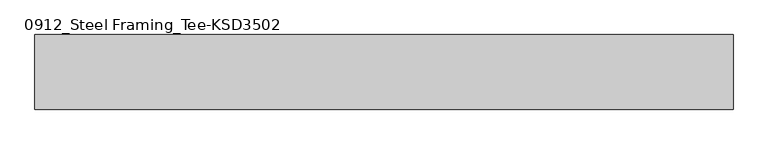
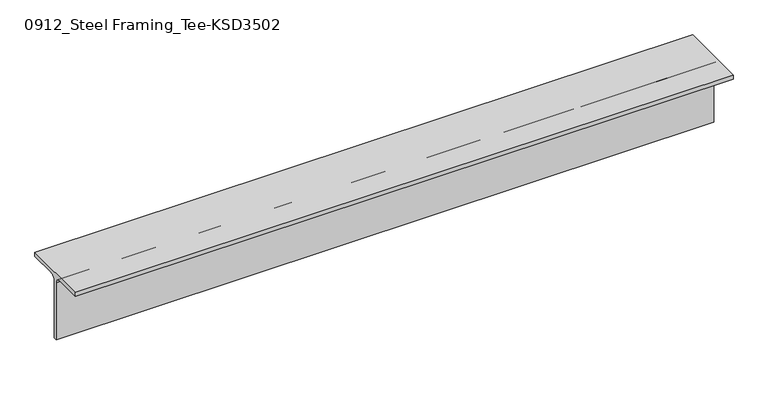
"""IFC4 building model written with IfcOpenShell, lengths in millimetres: member geometry, 0912_Steel Framing_Tee-KSD3502 : H_SB_ASB_CT-150x150x6.5x9."""

from ifc_helpers import new_model, si_unit, point, frame, frame_2d, origin, place, context, project, spatial, polyline, circle_curve, trimmed, segment, composite_curve, outline, extrude, source, transform, mapped, element, save


def member_0912_steel_framing_tee_ksd3502_6a97d332(model_context):
    return source(origin(), model_context, "Body", "SweptSolid", [
        extrude(outline(composite_curve([segment(polyline([(75.0, 75.0), (75.0, 66.0), (16.25, 66.0)]), True, "CONTINUOUS"), segment(trimmed(circle_curve(frame_2d((16.25, 53.0)), 13.0), [point((16.25, 66.0))], [point((3.25, 53.0))], True, "CARTESIAN"), True, "CONTINUOUS"), segment(polyline([(3.25, 53.0), (3.25, -75.0), (-3.25, -75.0), (-3.25, 53.0)]), True, "CONTINUOUS"), segment(trimmed(circle_curve(frame_2d((-16.25, 53.0)), 13.0), [point((-3.25, 53.0))], [point((-16.25, 66.0))], True, "CARTESIAN"), True, "CONTINUOUS"), segment(polyline([(-16.25, 66.0), (-75.0, 66.0), (-75.0, 75.0), (75.0, 75.0)]), True, "CONTINUOUS")], self_intersect=False)), frame((-701.75, 0.0, 0.0), z_axis=(1.0, 0.0, 0.0), x_axis=(0.0, 1.0, 0.0)), (0.0, 0.0, 1.0), 1403.5),
    ])


if __name__ == "__main__":
    model = new_model("IFC4")
    model_context = context("Model", 3, world=origin())
    ifc_project = project(units=[si_unit("LENGTHUNIT", "METRE", prefix="MILLI")], contexts=[model_context])
    site = spatial("IfcSite", under=ifc_project)
    building = spatial("IfcBuilding", under=site)
    placement = place(None, origin())
    member_0912_steel_framing_tee_ksd3502_shape = member_0912_steel_framing_tee_ksd3502_6a97d332(model_context)
    element("IfcMember", 1, ObjectType="0912_Steel Framing_Tee-KSD3502 : H_SB_ASB_CT-150x150x6.5x9", at=placement, inside=building, context=model_context, shape_type="MappedRepresentation", body=[
        mapped(member_0912_steel_framing_tee_ksd3502_shape, transform((0.0, 0.0, 0.0), x_axis=(1.0, 0.0, 0.0), y_axis=(0.0, 1.0, 0.0), z_axis=(0.0, 0.0, 1.0))),
    ])
    save(model, "model.ifc")

# Revit data of these elements
# Type "0912_Steel Framing_Tee-KSD3502 : H_SB_ASB_CT-150x150x6.5x9"
#   H_WM Code_1 = "S01AA003-00001 | Main Steel Structure Fabrication Work | Shelter/Building | Light Steel - Standard (30KG/M>Weight) | Material: (   )"
#   H_WM Code_2 = "S03AA029-00001 | Main Steel Structure Erection Work | Shelter/Building | Light Steel (30KG/M>Weight) | Material: (   )"
#   H_WM Code_3 = "S01AA010-00001 | Main Steel Structure Fabrication Work | Shelter/Building | Steel Painting/Coating | for Non-Fireproofed Steel Surface, Surface Preparation, Primer, Second & Final Coat | Material: (   )"
#   H_Q'ty Cal Type Tag = "SB-Q2"
#   Width = 15.0 cm
#   Web Thickness = 0.65 cm
#   Web Fillet = 1.3 cm
#   Section Area = 23.39 cm²
#   Perimeter = 0.60 m²/m
#   Nominal Weight = 18.40 kgf/m
#   Height = 15.0 cm
#   Flange Thickness = 0.9 cm
#   Centroid Vertical = 7.5 cm
#   Centroid Horizontal = 7.5 cm
#   Length [instance default] = 1.5000 m
#   Structural Material [instance default] = Steel, 45-345
#   Warping Constant = (empty or 0)
#   Torsional Moment of Inertia = 0
#   Section Name Key = ""
#   Plastic Modulus weak axis = 0
#   Plastic Modulus strong axis = 0
#   Moment of Inertia weak axis = 0
#   Moment of Inertia strong axis = 0
#   Elastic Modulus weak axis = 0
#   Elastic Modulus strong axis = 0
#   Bolt Spacing = 0
#   Assembly Code = ""
# Element 1 (IfcMember, "0912_Steel Framing_Tee-KSD3502 : H_SB_ASB_CT-150x150x6.5x9")
#   Structural Material = none
# Materials
#   "Steel, 45-345": class "Metal", colour RGB 189 187 185, transparency 0, Description = "Steel 345 MPa", Cost = 0
